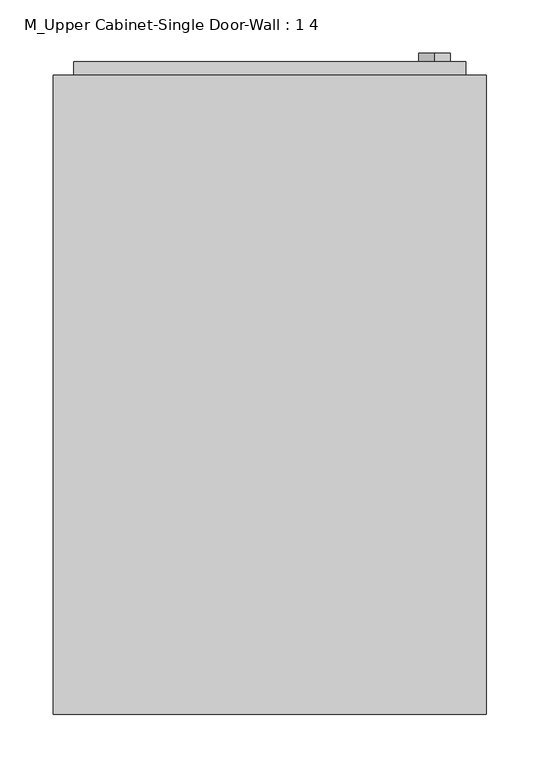
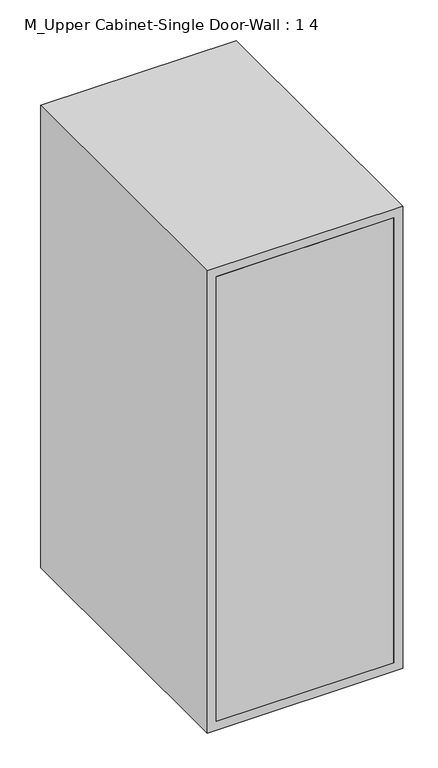
"""IFC4 building model written with IfcOpenShell, lengths in millimetres: furniture geometry, M_Upper Cabinet-Single Door-Wall : 1 4."""

from ifc_helpers import new_model, si_unit, point, frame, frame_2d, origin, place, context, project, spatial, polyline, circle_curve, trimmed, segment, composite_curve, outline, extrude, source, transform, mapped, element, save


def m_upper_cabinet_single_door_wall_1_4_e3706d9b(model_context):
    return source(origin(), model_context, "Body", "SweptSolid", [
        extrude(outline(polyline([(-154.3788372, 669.8257813), (213.9211628, 669.8257813), (213.9211628, 638.0757813), (-154.3788372, 638.0757813), (-154.3788372, 669.8257813)])), frame((0.0, 0.0, 1003.05), z_axis=(0.0, 0.0, 1.0), x_axis=(1.0, 0.0, 0.0)), (0.0, 0.0, 1.0), 977.9),
        extrude(outline(polyline([(213.9211628, 57.15), (-154.3788372, 57.15), (-154.3788372, 76.2), (213.9211628, 76.2), (213.9211628, 57.15)])), frame((0.0, 0.0, 1003.05), z_axis=(0.0, 0.0, 1.0), x_axis=(1.0, 0.0, 0.0)), (0.0, 0.0, 1.0), 977.9),
        extrude(outline(polyline([(2000.0, -173.4288372), (984.0, -173.4288372), (984.0, 232.9711628), (2000.0, 232.9711628), (2000.0, -173.4288372)]), holes=[polyline([(1980.95, -154.3788372), (1980.95, 213.9211628), (1003.05, 213.9211628), (1003.05, -154.3788372), (1980.95, -154.3788372)])]), frame((0.0, 57.15, 0.0), z_axis=(0.0, 1.0, 0.0), x_axis=(0.0, 0.0, 1.0)), (0.0, 0.0, 1.0), 599.9757812),
        extrude(outline(composite_curve([segment(trimmed(circle_curve(frame_2d((1179.0953371, 184.3613252)), 15.0), [point((1164.0953371, 184.3613252))], [point((1194.0953371, 184.3613252))], False, "CARTESIAN"), True, "CONTINUOUS"), segment(trimmed(circle_curve(frame_2d((1179.0953371, 184.3613252)), 15.0), [point((1194.0953371, 184.3613252))], [point((1164.0953371, 184.3613252))], False, "CARTESIAN"), True, "CONTINUOUS")], self_intersect=False)), frame((0.0, 669.8257813, 0.0), z_axis=(0.0, 1.0, 0.0), x_axis=(0.0, 0.0, 1.0)), (0.0, 0.0, 1.0), 8.0),
    ])


if __name__ == "__main__":
    model = new_model("IFC4")
    model_context = context("Model", 3, world=origin())
    ifc_project = project(units=[si_unit("LENGTHUNIT", "METRE", prefix="MILLI")], contexts=[model_context])
    site = spatial("IfcSite", under=ifc_project)
    building = spatial("IfcBuilding", under=site)
    placement = place(None, origin())
    m_upper_cabinet_single_door_wall_1_4_shape = m_upper_cabinet_single_door_wall_1_4_e3706d9b(model_context)
    element("IfcFurniture", 1, ObjectType="M_Upper Cabinet-Single Door-Wall : 1 4", at=placement, inside=building, context=model_context, shape_type="MappedRepresentation", body=[
        mapped(m_upper_cabinet_single_door_wall_1_4_shape, transform((0.0, 0.0, 0.0), x_axis=(1.0, 0.0, 0.0), y_axis=(0.0, 1.0, 0.0), z_axis=(0.0, 0.0, 1.0))),
    ])
    save(model, "model.ifc")

# Revit data of these elements
# Type "M_Upper Cabinet-Single Door-Wall : 1 4"
#   Depth = 1' - 11 159/256"
#   Height = 3' - 4"
#   Top Of Cabinet = 6' - 6.74016"
#   Width = 1' - 4"
#   Cabinet Material = Base cabinet 2120100 Aspekt - 83012120100 - White
#   Door/Drawer Material = Base cabinet 2120100 Aspekt - 83012120100 - White
#   Handle Material = Cabinets - Handles
#   Default Elevation = 0
# Element 1 (IfcFurniture, "M_Upper Cabinet-Single Door-Wall : 1 4")
#   Materials on its faces: "Base cabinet 2120100 Aspekt - 83012120100 - White"
# Materials
#   "Base cabinet 2120100 Aspekt - 83012120100 - White": class "Miscellaneous", colour RGB 255 255 255, transparency 0, Manufacturer = "Marbodal", URL = "http://www.marbodal.se", Cost = 0
#   "Cabinets - Handles": class "Metal", colour RGB 57 57 57, transparency 0
